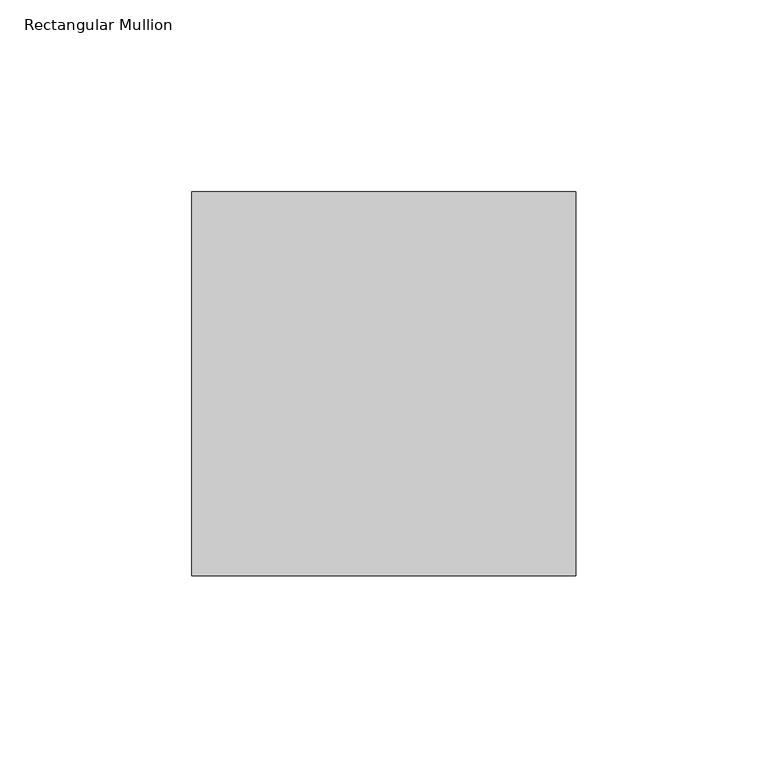
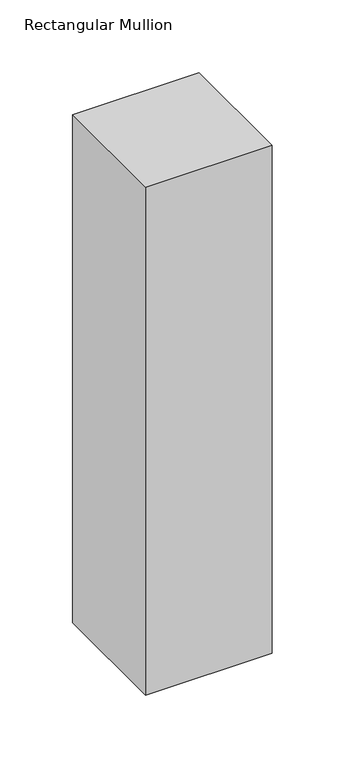
"""IFC4 building model written with IfcOpenShell, lengths in millimetres: member geometry, Rectangular Mullion : 알루미늄_Rectangular Cap_100 x100."""

from ifc_helpers import new_model, si_unit, frame, origin, place, context, project, spatial, polyline, outline, extrude, source, transform, mapped, element, save


def rectangular_mullion_bd602285(model_context):
    return source(origin(), model_context, "Body", "SweptSolid", [
        extrude(outline(polyline([(0.0, 50.0), (0.0, -50.0), (-100.0, -50.0), (-100.0, 50.0), (0.0, 50.0)])), frame((0.0, 0.0, -425.0), z_axis=(0.0, 0.0, 1.0), x_axis=(1.0, 0.0, 0.0)), (0.0, 0.0, 1.0), 425.0),
    ])


if __name__ == "__main__":
    model = new_model("IFC4")
    model_context = context("Model", 3, world=origin())
    ifc_project = project(units=[si_unit("LENGTHUNIT", "METRE", prefix="MILLI")], contexts=[model_context])
    site = spatial("IfcSite", under=ifc_project)
    building = spatial("IfcBuilding", under=site)
    placement = place(None, origin())
    rectangular_mullion_shape = rectangular_mullion_bd602285(model_context)
    element("IfcMember", 1, ObjectType="Rectangular Mullion : 알루미늄_Rectangular Cap_100 x100", at=placement, inside=building, context=model_context, shape_type="MappedRepresentation", body=[
        mapped(rectangular_mullion_shape, transform((0.0, 0.0, 0.0), x_axis=(1.0, 0.0, 0.0), y_axis=(0.0, 1.0, 0.0), z_axis=(0.0, 0.0, 1.0))),
    ])
    save(model, "model.ifc")

# Revit data of these elements
# Type "Rectangular Mullion : 알루미늄_Rectangular Cap_100 x100"
#   built-in parameter 1007304 = 0.328084 (stored number, unit not read)
#   built-in parameter 1007301 = 0.164042 (stored number, unit not read)
#   built-in parameter 1007300 = 0.164042 (stored number, unit not read)
# Element 1 (IfcMember, "Rectangular Mullion : 알루미늄_Rectangular Cap_100 x100")
#   Materials on its faces: "00_Metal_Stainless Steel"
# Materials
#   "00_Metal_Stainless Steel": class "Metal", colour RGB 148 148 148, transparency 0, Description = "Steel", Cost = 0
